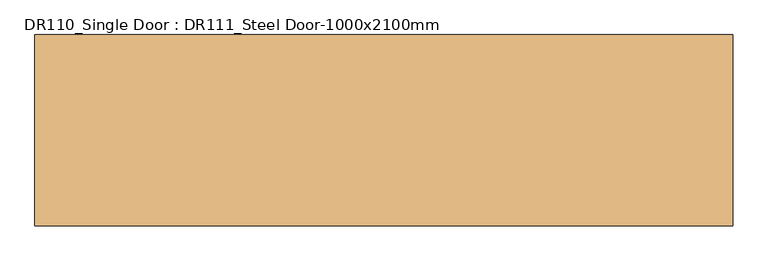
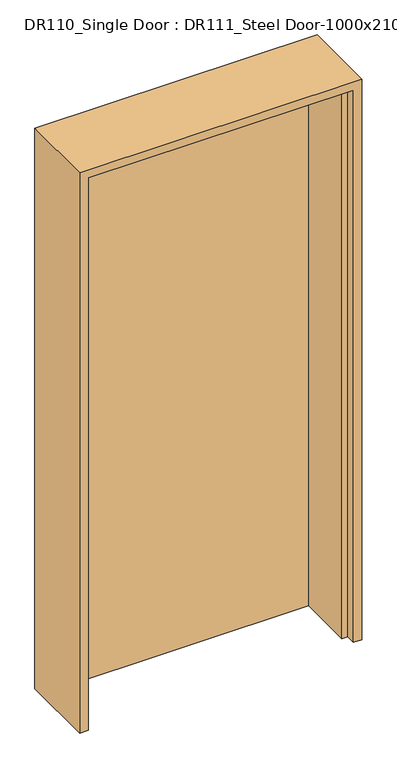
"""IFC4 building model written with IfcOpenShell, lengths in millimetres: door geometry, DR110_Single Door : DR111_Steel Door-1000x2100mm."""

from ifc_helpers import new_model, si_unit, origin, origin_with_axes, place, context, project, spatial, polyline, outline, extrude, faceted_brep, source, transform, mapped, element, save


def dr110_single_door_dr111_steel_door_1000x2100mm_d0b51d4b(model_context):
    return source(origin(), model_context, "Body", "SolidModel", [
        extrude(outline(polyline([(470.0, 137.0), (470.0, 102.0), (-470.0, 102.0), (-470.0, 137.0), (470.0, 137.0)])), origin_with_axes(), (0.0, 0.0, 1.0), 2070.0),
        faceted_brep([(470.0, 137.0, 0.0), (500.0, 137.0, 0.0), (500.0, -137.0, 0.0), (470.0, -137.0, 0.0), (470.0, -102.0, 0.0), (450.0, -102.0, 0.0), (450.0, 102.0, 0.0), (470.0, 102.0, 0.0), (470.0, 137.0, 2070.0), (-470.0, 137.0, 2070.0), (-470.0, 137.0, 0.0), (-500.0, 137.0, 0.0), (-500.0, 137.0, 2100.0), (500.0, 137.0, 2100.0), (500.0, -137.0, 2100.0), (-500.0, -137.0, 2100.0), (-500.0, -137.0, 0.0), (-470.0, -137.0, 0.0), (-470.0, -137.0, 2070.0), (470.0, -137.0, 2070.0), (470.0, -102.0, 2070.0), (-470.0, -102.0, 2070.0), (-470.0, -102.0, 0.0), (-450.0, -102.0, 0.0), (-450.0, -102.0, 2050.0), (450.0, -102.0, 2050.0), (450.0, 102.0, 2050.0), (-450.0, 102.0, 2050.0), (-450.0, 102.0, 0.0), (-470.0, 102.0, 0.0), (-470.0, 102.0, 2070.0), (470.0, 102.0, 2070.0)], [[[0, 1, 2, 3, 4, 5, 6, 7]], [[1, 0, 8, 9, 10, 11, 12, 13]], [[2, 1, 13, 14]], [[3, 2, 14, 15, 16, 17, 18, 19]], [[4, 3, 19, 20]], [[5, 4, 20, 21, 22, 23, 24, 25]], [[6, 5, 25, 26]], [[7, 6, 26, 27, 28, 29, 30, 31]], [[0, 7, 31, 8]], [[9, 30, 29, 10]], [[10, 29, 28, 23, 22, 17, 16, 11]], [[15, 12, 11, 16]], [[21, 18, 17, 22]], [[27, 24, 23, 28]], [[14, 13, 12, 15]], [[20, 19, 18, 21]], [[26, 25, 24, 27]], [[8, 31, 30, 9]]]),
    ])


if __name__ == "__main__":
    model = new_model("IFC4")
    model_context = context("Model", 3, world=origin())
    ifc_project = project(units=[si_unit("LENGTHUNIT", "METRE", prefix="MILLI")], contexts=[model_context])
    site = spatial("IfcSite", under=ifc_project)
    building = spatial("IfcBuilding", under=site)
    placement = place(None, origin())
    dr110_single_door_dr111_steel_door_1000x2100mm_shape = dr110_single_door_dr111_steel_door_1000x2100mm_d0b51d4b(model_context)
    element("IfcDoor", 1, ObjectType="DR110_Single Door : DR111_Steel Door-1000x2100mm", at=placement, inside=building, context=model_context, shape_type="MappedRepresentation", body=[
        mapped(dr110_single_door_dr111_steel_door_1000x2100mm_shape, transform((0.0, 0.0, 0.0), x_axis=(1.0, 0.0, 0.0), y_axis=(0.0, 1.0, 0.0), z_axis=(0.0, 0.0, 1.0))),
    ])
    save(model, "model.ifc")

# Revit data of these elements
# Type "DR110_Single Door : DR111_Steel Door-1000x2100mm"
#   Type Mark = "SD"
#   Analytic Construction = "<None>"
#   프레임 투영 외부. = 25 mm
#   프레임 투영 내부. = 25 mm
#   프레임 폭 = 75 mm
#   Height = 2100 mm
#   Width = 1000 mm
#   Define Thermal Properties by = 1
#   문 패널 = SD1 문 패널
#   문 프레임 = A04AQ098-00002_Steel Door_non FP_single
#   Function = (empty or 0)
#   Wall Closure = (empty or 0)
# Element 1 (IfcDoor, "DR110_Single Door : DR111_Steel Door-1000x2100mm")
#   Materials on its faces: "A04AQ098-00002_Steel Door_non FP_single", "SD1 문 패널"
# Materials
#   "SD1 문 패널": class "금속", colour RGB 247 247 247, transparency 0, Description = "STEEL DOOR (1000Wx2100H)"
#   "A04AQ098-00002_Steel Door_non FP_single": class "금속", colour RGB 247 247 247, transparency 0, Description = "Steel Door", W00) Work Master Code = "A04AQ098-00002", W01) Work Master_Lv1 = "Finishing Work", W02) Work Master_Lv2 = "Door & Window Work", W03) Work Master_Spec.1 = "Steel Door w/ Steel Frame", W04) Work Master_Spec.2 = "Fire Protective Rating: N/A, Single Door", W05) Work Master_Spec.3 = "w/ Hardware & Accessories", Cost = 0
